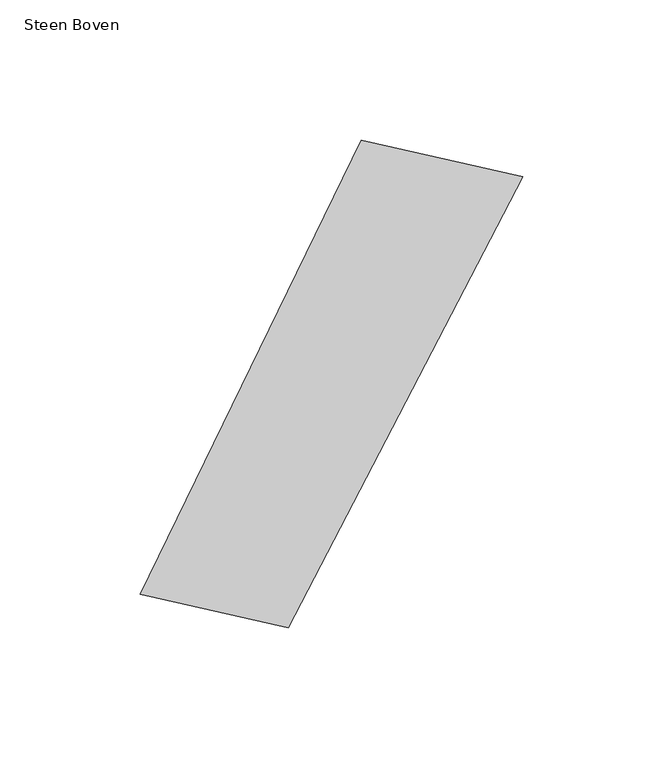
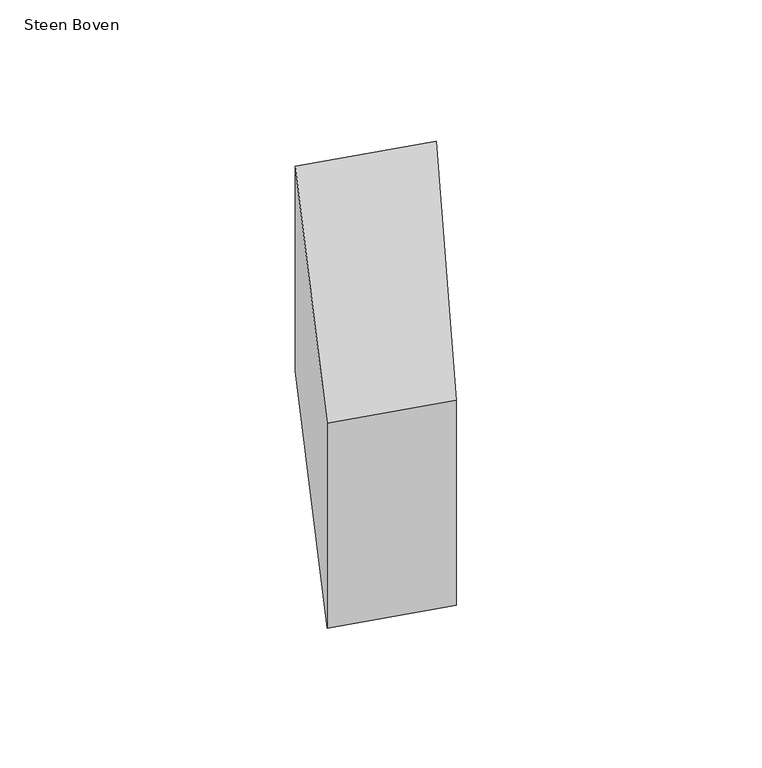
"""IFC4 building model written with IfcOpenShell, lengths in millimetres: proxy geometry, 00_GMA_steen_versie_4 : Steen Boven."""

from ifc_helpers import new_model, si_unit, origin, origin_with_axes, place, context, project, spatial, polyline, outline, extrude, source, transform, mapped, element, save


def steen_boven_6e46f58c(model_context):
    return source(origin(), model_context, "Body", "SweptSolid", [
        extrude(outline(polyline([(143.5582911, 152.2686047), (60.0999612, -8.4277022), (7.3163998, 3.5526856), (86.0489792, 165.2920935), (143.5582911, 152.2686047)])), origin_with_axes(), (0.0, 0.0, 1.0), 100.0),
    ])


if __name__ == "__main__":
    model = new_model("IFC4")
    model_context = context("Model", 3, world=origin())
    ifc_project = project(units=[si_unit("LENGTHUNIT", "METRE", prefix="MILLI")], contexts=[model_context])
    site = spatial("IfcSite", under=ifc_project)
    building = spatial("IfcBuilding", under=site)
    placement = place(None, origin())
    steen_boven_shape = steen_boven_6e46f58c(model_context)
    element("IfcBuildingElementProxy", 1, Name="00_GMA_steen_versie_4 : Steen Boven", ObjectType="00_GMA_steen_versie_4 : Steen Boven", at=placement, inside=building, context=model_context, shape_type="MappedRepresentation", body=[
        mapped(steen_boven_shape, transform((0.0, 0.0, 0.0), x_axis=(1.0, 0.0, 0.0), y_axis=(0.0, 1.0, 0.0), z_axis=(0.0, 0.0, 1.0))),
    ])
    save(model, "model.ifc")

# Revit data of these elements
# Type "00_GMA_steen_versie_4 : Steen Boven"
#   StootVoegHalfBoven [instance default] = 5 mm
#   StootVoegHalf [instance default] = 5 mm
#   StootVoegBreedteOnder = 10 mm
#   StootVoegBreedteBoven = 10 mm
#   Steendikte = 100 mm
#   LintVoegOnderHalf = 5 mm
#   LintVoegOnder = 10 mm
#   LintVoegBovenHalf = 0 mm
#   LintVoegBoven = 0 mm
#   materiaal = none
#   MateriaalVoeg = none
#   Default Elevation = 0
